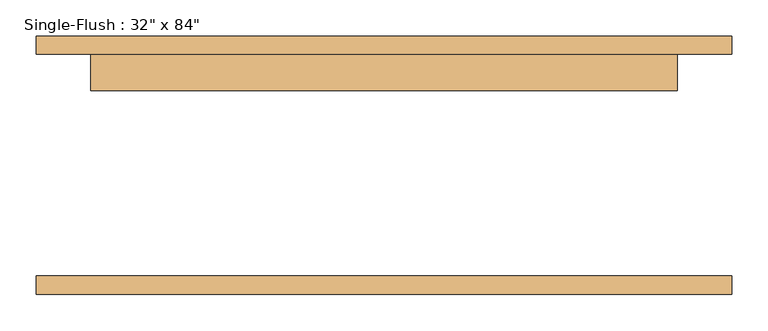
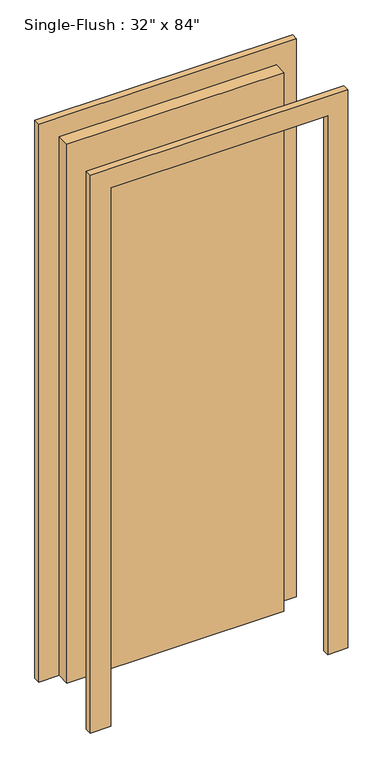
"""IFC4 building model written with IfcOpenShell, lengths in millimetres: door geometry."""

from ifc_helpers import new_model, si_unit, frame, origin, origin_with_axes, place, context, project, spatial, polyline, outline, extrude, source, transform, mapped, element, save


def door_e8108b55(model_context):
    return source(origin(), model_context, "Body", "SweptSolid", [
        extrude(outline(polyline([(2209.8, -482.6), (0.0, -482.6), (0.0, -406.4), (2133.6, -406.4), (2133.6, 406.4), (0.0, 406.4), (0.0, 482.6), (2209.8, 482.6), (2209.8, -482.6)])), frame((0.0, 153.9875, 0.0), z_axis=(0.0, 1.0, 0.0), x_axis=(0.0, 0.0, 1.0)), (0.0, 0.0, 1.0), 25.4),
        extrude(outline(polyline([(2209.8, 482.6), (2209.8, -482.6), (0.0, -482.6), (0.0, -406.4), (2133.6, -406.4), (2133.6, 406.4), (0.0, 406.4), (0.0, 482.6), (2209.8, 482.6)])), frame((0.0, -179.3875, 0.0), z_axis=(0.0, 1.0, 0.0), x_axis=(0.0, 0.0, 1.0)), (0.0, 0.0, 1.0), 25.4),
        extrude(outline(polyline([(406.4, 103.1875), (-406.4, 103.1875), (-406.4, 153.9875), (406.4, 153.9875), (406.4, 103.1875)])), origin_with_axes(), (0.0, 0.0, 1.0), 2133.6),
    ])


if __name__ == "__main__":
    model = new_model("IFC4")
    model_context = context("Model", 3, world=origin())
    ifc_project = project(units=[si_unit("LENGTHUNIT", "METRE", prefix="MILLI")], contexts=[model_context])
    site = spatial("IfcSite", under=ifc_project)
    building = spatial("IfcBuilding", under=site)
    placement = place(None, origin())
    door_shape = door_e8108b55(model_context)
    element("IfcDoor", 1, ObjectType="Single-Flush : 32\" x 84\"", at=placement, inside=building, context=model_context, shape_type="MappedRepresentation", body=[
        mapped(door_shape, transform((0.0, 0.0, 0.0), x_axis=(1.0, 0.0, 0.0), y_axis=(0.0, 1.0, 0.0), z_axis=(0.0, 0.0, 1.0))),
    ])
    save(model, "model.ifc")

# Revit data of these elements
# Type "Single-Flush : 32\" x 84\""
#   Type Mark = "10"
#   Construction Type Id = "MDOOR"
#   Assembly Code = "C1020"
#   Analytic Construction = "Metal"
#   Thickness = 0' - 2"
#   Heat Transfer Coefficient (U) = 3.7021 W/(m²·K)
#   Height = 7' - 0"
#   Trim Projection Ext = 0' - 1"
#   Trim Projection Int = 0' - 1"
#   Trim Width = 0' - 3"
#   Width = 2' - 8"
#   Door Material = Door - Panel
#   Frame Material = Door - Frame
#   Visual Light Transmittance = 0
#   Solar Heat Gain Coefficient = 0
#   Function = (empty or 0)
#   Wall Closure = (empty or 0)
# Element 1 (IfcDoor, "Single-Flush : 32\" x 84\"")
#   Materials on its faces: "Door - Frame", "Door - Panel"
# Materials
#   "Door - Panel": class "Wood", colour RGB 210 159 95, transparency 0
#   "Door - Frame": class "Miscellaneous", colour RGB 118 70 51, transparency 0
